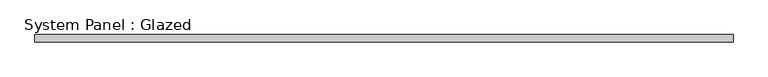
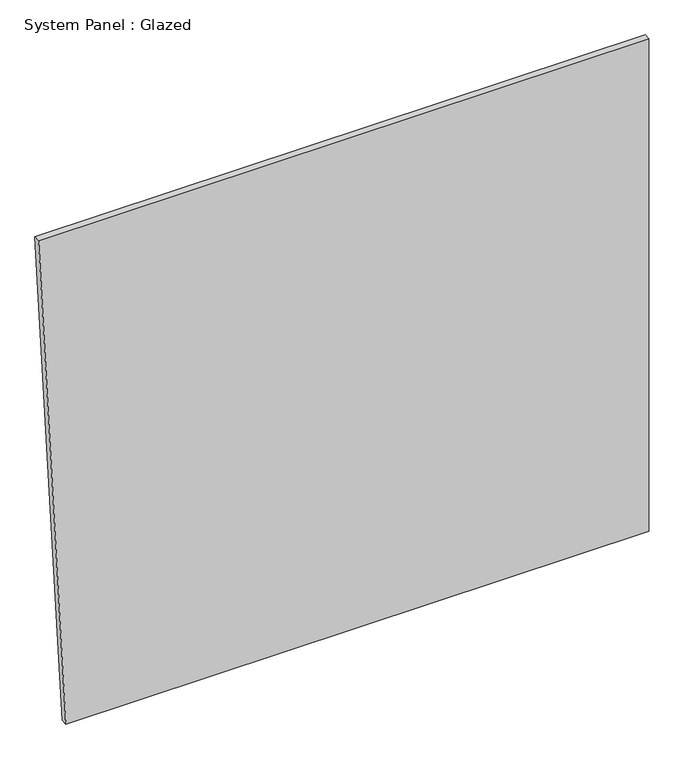
"""IFC4 building model written with IfcOpenShell, lengths in millimetres: plate geometry, System Panel : Glazed."""

from ifc_helpers import new_model, si_unit, frame, origin, place, context, project, spatial, polyline, outline, extrude, source, transform, mapped, element, save


def system_panel_glazed_bdf74c23(model_context):
    return source(origin(), model_context, "Body", "SweptSolid", [
        extrude(outline(polyline([(0.0, -1112.8894655), (0.0, 1222.0297486), (2085.3785982, 1222.0297486), (2085.3785982, -1222.0297486), (0.0, -1112.8894655)])), frame((0.0, -44.45, 0.0), z_axis=(0.0, 1.0, 0.0), x_axis=(0.0, 0.0, 1.0)), (0.0, 0.0, 1.0), 25.4),
    ])


if __name__ == "__main__":
    model = new_model("IFC4")
    model_context = context("Model", 3, world=origin())
    ifc_project = project(units=[si_unit("LENGTHUNIT", "METRE", prefix="MILLI")], contexts=[model_context])
    site = spatial("IfcSite", under=ifc_project)
    building = spatial("IfcBuilding", under=site)
    placement = place(None, origin())
    system_panel_glazed_shape = system_panel_glazed_bdf74c23(model_context)
    element("IfcPlate", 1, ObjectType="System Panel : Glazed", at=placement, inside=building, context=model_context, shape_type="MappedRepresentation", body=[
        mapped(system_panel_glazed_shape, transform((0.0, 0.0, 0.0), x_axis=(1.0, 0.0, 0.0), y_axis=(0.0, 1.0, 0.0), z_axis=(0.0, 0.0, 1.0))),
    ])
    save(model, "model.ifc")

# Revit data of these elements
# Type "System Panel : Glazed"
#   Construction Type Id = "GSP4R"
#   Analytic Construction = "1/8 in Pilkington single glazing"
#   Visual Light Transmittance = 0.9
#   Solar Heat Gain Coefficient = 0.86
#   Heat Transfer Coefficient (U) = 1.18115 BTU/(h·ft²·°F)
#   Define Thermal Properties by = 1
# Element 1 (IfcPlate, "System Panel : Glazed")
#   Materials on its faces: "Glass"
# Materials
#   "Glass": class "Glass", colour RGB 0 128 192, transparency 0.75, Description = "Soda Lime Glass", Cost = 0
